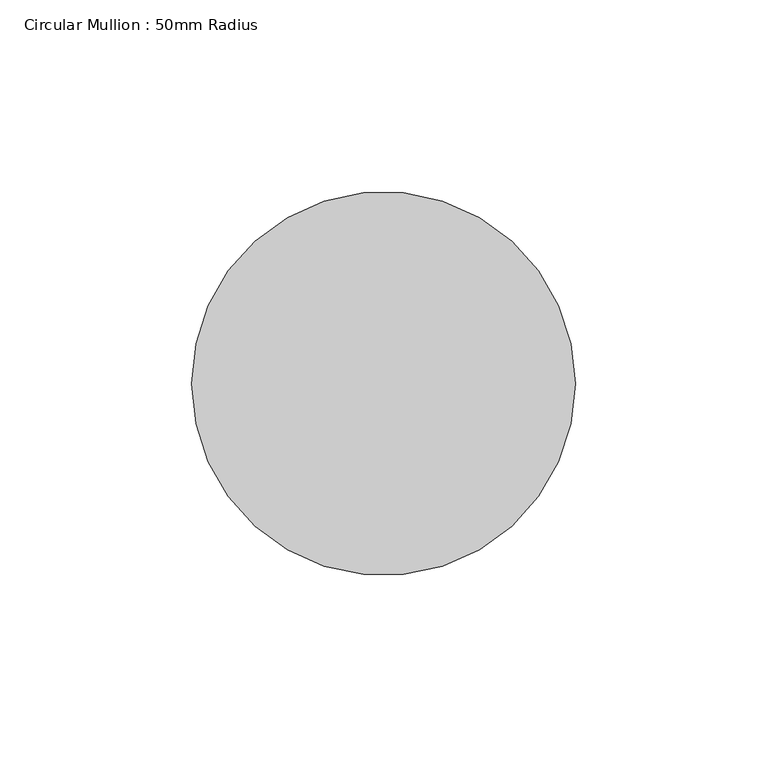
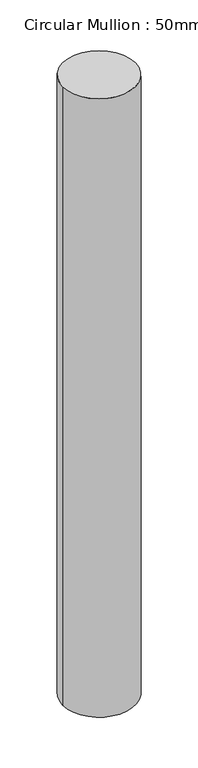
"""IFC4 building model written with IfcOpenShell, lengths in millimetres: member geometry, Circular Mullion : 50mm Radius."""

import ifcopenshell
import ifcopenshell.guid

model = None  # the IFC model being written
_history = None  # IfcOwnerHistory: only IFC2X3 demands one
_inside = {}  # id of a spatial element -> (the spatial element, [elements in it])
_under = {}  # id of a project, library or spatial element -> (it, [spatial elements below it])
_declared = {}  # id of a project -> (the project, [libraries it declares])
_typed = {}  # id of a type object -> (the type object, [elements of that type])
_made_of = {}  # id of a material, layer set ... -> (it, [elements and type objects made of it])


def new_model(schema):
    """Start an empty IFC model of exactly this schema.

    Asked for "IFC4X3", IfcOpenShell would pick the latest addendum, in which some entities
    have other attributes; the version numbers below select the first issue.
    IFC2X3 requires an IfcOwnerHistory on every rooted entity: one is made here for all.
    """
    global model, _history
    if schema == "IFC4X3":
        model = ifcopenshell.file(schema_version=(4, 3, 0, 0))
    else:
        model = ifcopenshell.file(schema=schema)
    _inside.clear()
    _under.clear()
    _declared.clear()
    _typed.clear()
    _made_of.clear()
    _history = None
    if model.schema == "IFC2X3":
        org = make("IfcOrganization", Name="unknown")
        user = make(
            "IfcPersonAndOrganization",
            ThePerson=make("IfcPerson", FamilyName="unknown"),
            TheOrganization=org,
        )
        app = make(
            "IfcApplication",
            ApplicationDeveloper=org,
            Version="unknown",
            ApplicationFullName="unknown",
            ApplicationIdentifier="unknown",
        )
        _history = make(
            "IfcOwnerHistory",
            OwningUser=user,
            OwningApplication=app,
            ChangeAction="ADDED",
            CreationDate=0,
        )
    return model


def make(cls, **values):
    """One entity of the class cls with the attributes given. An attribute that is None is left unset."""
    return model.create_entity(
        cls, **{name: value for name, value in values.items() if value is not None}
    )


def rooted(cls, **values):
    """An entity with a GlobalId (a new one), such as an element, a storey or a relation."""
    return make(cls, GlobalId=ifcopenshell.guid.new(), OwnerHistory=_history, **values)


def si_unit(unit_type, name, prefix=None):
    """IfcSIUnit, for example si_unit("LENGTHUNIT", "METRE", prefix="MILLI")."""
    return make("IfcSIUnit", UnitType=unit_type, Prefix=prefix, Name=name)


def assignment(units):
    """IfcUnitAssignment: the units of a project."""
    return None if units is None else make("IfcUnitAssignment", Units=units)


def point(xyz):
    """IfcCartesianPoint."""
    return None if xyz is None else make("IfcCartesianPoint", Coordinates=xyz)


def direction(xyz):
    """IfcDirection."""
    return None if xyz is None else make("IfcDirection", DirectionRatios=xyz)


def frame(location, z_axis=None, x_axis=None):
    """IfcAxis2Placement3D, a coordinate frame: its origin and axes. An axis left out is left unset."""
    return make(
        "IfcAxis2Placement3D",
        Location=point(location),
        Axis=direction(z_axis),
        RefDirection=direction(x_axis),
    )


def frame_2d(location, x_axis=None):
    """IfcAxis2Placement2D, a coordinate frame in the plane: its origin and x axis."""
    return make(
        "IfcAxis2Placement2D", Location=point(location), RefDirection=direction(x_axis)
    )


def origin():
    """The frame at (0, 0, 0) with its axes left unset."""
    return frame((0.0, 0.0, 0.0))


def origin_2d():
    """The frame at (0, 0) in the plane with its x axis left unset."""
    return frame_2d((0.0, 0.0))


def place(relative_to, where):
    """IfcLocalPlacement: puts the frame where relative to a parent placement (None: the world)."""
    return make(
        "IfcLocalPlacement", PlacementRelTo=relative_to, RelativePlacement=where
    )


def context(
    kind, dimensions, precision=None, world=None, true_north=None, identifier=None
):
    """IfcGeometricRepresentationContext, for example the 3D "Model" context."""
    return make(
        "IfcGeometricRepresentationContext",
        ContextIdentifier=identifier,
        ContextType=kind,
        CoordinateSpaceDimension=dimensions,
        Precision=precision,
        WorldCoordinateSystem=world,
        TrueNorth=true_north,
    )


def project(units=None, contexts=None):
    """IfcProject with its units and contexts."""
    return rooted(
        "IfcProject",
        Name="project",
        RepresentationContexts=contexts,
        UnitsInContext=assignment(units),
    )


def spatial(cls, under=None, at=None, **own):
    """A site, building, storey or space (cls), placed at a placement, below another one or the project."""
    s = rooted(cls, ObjectPlacement=at, **own)
    if under is not None:
        _under.setdefault(under.id(), (under, []))[1].append(s)
    return s


def circle_curve(where, radius):
    """IfcCircle in the frame where."""
    return make("IfcCircle", Position=where, Radius=radius)


def trimmed(basis, trim1, trim2, sense, master):
    """IfcTrimmedCurve: the piece of a basis curve between two trims."""
    return make(
        "IfcTrimmedCurve",
        BasisCurve=basis,
        Trim1=trim1,
        Trim2=trim2,
        SenseAgreement=sense,
        MasterRepresentation=master,
    )


def segment(curve, same_sense, transition):
    """IfcCompositeCurveSegment."""
    return make(
        "IfcCompositeCurveSegment",
        Transition=transition,
        SameSense=same_sense,
        ParentCurve=curve,
    )


def composite_curve(segments, self_intersect=None):
    """IfcCompositeCurve: segments joined end to end."""
    return make("IfcCompositeCurve", Segments=segments, SelfIntersect=self_intersect)


def outline(outer, holes=None, kind="AREA"):
    """IfcArbitraryClosedProfileDef: a profile drawn as a closed curve; with holes, ...WithVoids."""
    if holes is None:
        return make("IfcArbitraryClosedProfileDef", ProfileType=kind, OuterCurve=outer)
    return make(
        "IfcArbitraryProfileDefWithVoids",
        ProfileType=kind,
        OuterCurve=outer,
        InnerCurves=holes,
    )


def extrude(swept, where, along, depth):
    """IfcExtrudedAreaSolid: the profile swept, set in the frame where, extruded along a direction by depth."""
    return make(
        "IfcExtrudedAreaSolid",
        SweptArea=swept,
        Position=where,
        ExtrudedDirection=direction(along),
        Depth=depth,
    )


def shape(context_of_items, identifier, shape_type, items):
    """IfcShapeRepresentation: the items that make up one representation, for example the "Body"."""
    return make(
        "IfcShapeRepresentation",
        ContextOfItems=context_of_items,
        RepresentationIdentifier=identifier,
        RepresentationType=shape_type,
        Items=items,
    )


def source(mapping_origin, context_of_items, identifier, shape_type, items):
    """IfcRepresentationMap: a shape defined once, which mapped items show again and again."""
    return make(
        "IfcRepresentationMap",
        MappingOrigin=mapping_origin,
        MappedRepresentation=shape(context_of_items, identifier, shape_type, items),
    )


def transform(
    local_origin,
    x_axis=None,
    y_axis=None,
    z_axis=None,
    scale=None,
    scale2=None,
    scale3=None,
    uniform=True,
):
    """IfcCartesianTransformationOperator3D, or its non-uniform kind. x_axis, y_axis, z_axis: its Axis1, 2, 3."""
    if uniform:
        return make(
            "IfcCartesianTransformationOperator3D",
            Axis1=direction(x_axis),
            Axis2=direction(y_axis),
            LocalOrigin=point(local_origin),
            Scale=scale,
            Axis3=direction(z_axis),
        )
    return make(
        "IfcCartesianTransformationOperator3DnonUniform",
        Axis1=direction(x_axis),
        Axis2=direction(y_axis),
        LocalOrigin=point(local_origin),
        Scale=scale,
        Axis3=direction(z_axis),
        Scale2=scale2,
        Scale3=scale3,
    )


def mapped(mapping_source, mapping_target):
    """IfcMappedItem: shows the shape of a source again, moved by a transform."""
    return make(
        "IfcMappedItem", MappingSource=mapping_source, MappingTarget=mapping_target
    )


def made_of(thing, what):
    """Note that an element or type object is made of a material, layer set ...; save() writes the relation."""
    if what is not None:
        _made_of.setdefault(what.id(), (what, []))[1].append(thing)
    return thing


def element(
    cls,
    number,
    at=None,
    inside=None,
    cuts=None,
    type_object=None,
    material=None,
    context=None,
    identifier="Body",
    shape_type=None,
    held_by="IfcProductDefinitionShape",
    body=None,
    shapes=None,
    **own,
):
    """One element of the class cls, such as IfcWall. Its Tag is "e" and its number.

    at: its placement. inside: the storey or other place that contains it. cuts: it is an
    opening in that element (IfcRelVoidsElement). A single representation is given by context,
    identifier, shape_type and body (its items); several are given by shapes. held_by: the class
    of the entity that holds the representations. save() writes the other relations.
    """
    e = rooted(cls, Tag="e%d" % number, ObjectPlacement=at, **own)
    if body is not None:
        shapes = [shape(context, identifier, shape_type, body)]
    if shapes is not None:
        e.Representation = make(held_by, Representations=shapes)
    if inside is not None:
        _inside.setdefault(inside.id(), (inside, []))[1].append(e)
    if cuts is not None:
        rooted(
            "IfcRelVoidsElement", RelatingBuildingElement=cuts, RelatedOpeningElement=e
        )
    if type_object is not None:
        _typed.setdefault(type_object.id(), (type_object, []))[1].append(e)
    return made_of(e, material)


def aggregate(whole, parts):
    """IfcRelAggregates: a whole, such as a stair, and the parts it consists of."""
    return rooted("IfcRelAggregates", RelatingObject=whole, RelatedObjects=parts)


def save(model, path):
    """Write the relations noted so far, then the file.

    IfcRelAggregates (storeys below a building ...), IfcRelContainedInSpatialStructure (elements
    in a storey), IfcRelDefinesByType, IfcRelAssociatesMaterial and IfcRelDeclares: one each for
    every whole, place, type object, material and project.
    """
    for whole, parts in _under.values():
        aggregate(whole, parts)
    for where, things in _inside.values():
        rooted(
            "IfcRelContainedInSpatialStructure",
            RelatedElements=things,
            RelatingStructure=where,
        )
    for kind, things in _typed.values():
        rooted("IfcRelDefinesByType", RelatedObjects=things, RelatingType=kind)
    for what, things in _made_of.values():
        rooted("IfcRelAssociatesMaterial", RelatedObjects=things, RelatingMaterial=what)
    for by, libraries in _declared.values():
        rooted("IfcRelDeclares", RelatingContext=by, RelatedDefinitions=libraries)
    model.write(path)


def circular_mullion_50mm_radius_466ea7af(model_context):
    return source(origin(), model_context, "Body", "SweptSolid", [
        extrude(outline(composite_curve([segment(trimmed(circle_curve(origin_2d(), 50.0), [point((50.0, 0.0))], [point((-50.0, 0.0))], False, "CARTESIAN"), True, "CONTINUOUS"), segment(trimmed(circle_curve(origin_2d(), 50.0), [point((-50.0, 0.0))], [point((50.0, 0.0))], False, "CARTESIAN"), True, "CONTINUOUS")], self_intersect=False)), frame((0.0, 0.0, -900.1086308), z_axis=(0.0, 0.0, 1.0), x_axis=(1.0, 0.0, 0.0)), (0.0, 0.0, 1.0), 900.1086308),
    ])


if __name__ == "__main__":
    model = new_model("IFC4")
    model_context = context("Model", 3, world=origin())
    ifc_project = project(units=[si_unit("LENGTHUNIT", "METRE", prefix="MILLI")], contexts=[model_context])
    site = spatial("IfcSite", under=ifc_project)
    building = spatial("IfcBuilding", under=site)
    placement = place(None, origin())
    circular_mullion_50mm_radius_shape = circular_mullion_50mm_radius_466ea7af(model_context)
    element("IfcMember", 1, ObjectType="Circular Mullion : 50mm Radius", at=placement, inside=building, context=model_context, shape_type="MappedRepresentation", body=[
        mapped(circular_mullion_50mm_radius_shape, transform((0.0, 0.0, 0.0), x_axis=(1.0, 0.0, 0.0), y_axis=(0.0, 1.0, 0.0), z_axis=(0.0, 0.0, 1.0))),
    ])
    save(model, "model.ifc")

# Revit data of these elements
# Type "Circular Mullion : 50mm Radius"
#   built-in parameter 1007350 = 0.164042 (stored number, unit not read)
# Element 1 (IfcMember, "Circular Mullion : 50mm Radius")
#   Materials on its faces: "Aluminium"
# Materials
#   "Aluminium": class "Metal", colour RGB 247 247 247, transparency 0, Description = "Aluminium 6061", Cost = 0
